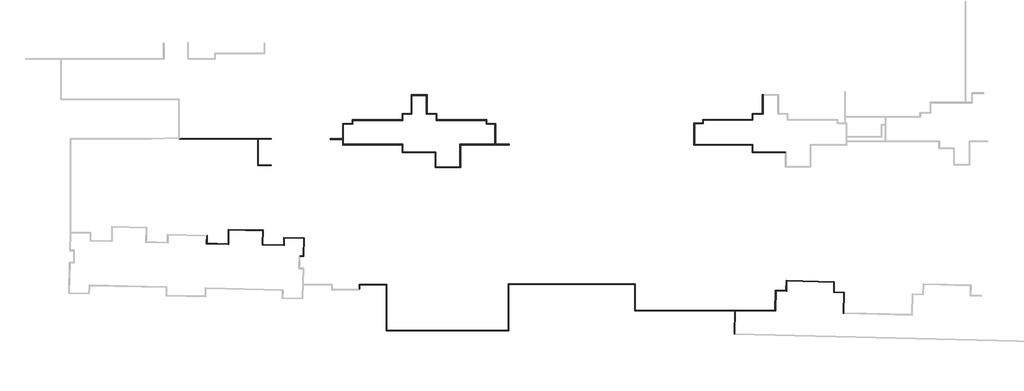
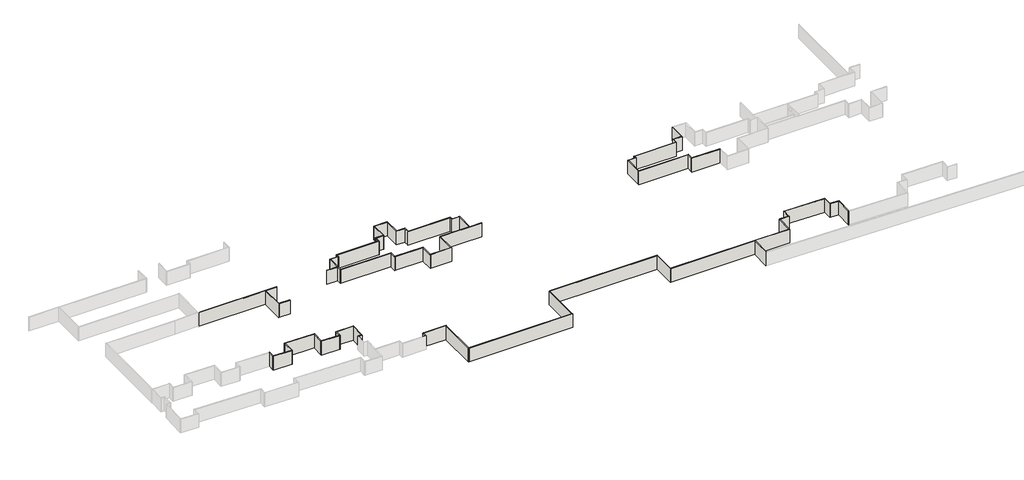
# One storey, part 2 of 8: 62 walls.
"""IFC4 building model written with IfcOpenShell, lengths in millimetres."""

import ifcopenshell
import ifcopenshell.guid

model = None  # the IFC model being written
_history = None  # IfcOwnerHistory: only IFC2X3 demands one
_inside = {}  # id of a spatial element -> (the spatial element, [elements in it])
_under = {}  # id of a project, library or spatial element -> (it, [spatial elements below it])
_declared = {}  # id of a project -> (the project, [libraries it declares])
_typed = {}  # id of a type object -> (the type object, [elements of that type])
_made_of = {}  # id of a material, layer set ... -> (it, [elements and type objects made of it])


def new_model(schema):
    """Start an empty IFC model of exactly this schema.

    Asked for "IFC4X3", IfcOpenShell would pick the latest addendum, in which some entities
    have other attributes; the version numbers below select the first issue.
    IFC2X3 requires an IfcOwnerHistory on every rooted entity: one is made here for all.
    """
    global model, _history
    if schema == "IFC4X3":
        model = ifcopenshell.file(schema_version=(4, 3, 0, 0))
    else:
        model = ifcopenshell.file(schema=schema)
    _inside.clear()
    _under.clear()
    _declared.clear()
    _typed.clear()
    _made_of.clear()
    _history = None
    if model.schema == "IFC2X3":
        org = make("IfcOrganization", Name="unknown")
        user = make(
            "IfcPersonAndOrganization",
            ThePerson=make("IfcPerson", FamilyName="unknown"),
            TheOrganization=org,
        )
        app = make(
            "IfcApplication",
            ApplicationDeveloper=org,
            Version="unknown",
            ApplicationFullName="unknown",
            ApplicationIdentifier="unknown",
        )
        _history = make(
            "IfcOwnerHistory",
            OwningUser=user,
            OwningApplication=app,
            ChangeAction="ADDED",
            CreationDate=0,
        )
    return model


def make(cls, **values):
    """One entity of the class cls with the attributes given. An attribute that is None is left unset."""
    return model.create_entity(
        cls, **{name: value for name, value in values.items() if value is not None}
    )


def rooted(cls, **values):
    """An entity with a GlobalId (a new one), such as an element, a storey or a relation."""
    return make(cls, GlobalId=ifcopenshell.guid.new(), OwnerHistory=_history, **values)


def si_unit(unit_type, name, prefix=None):
    """IfcSIUnit, for example si_unit("LENGTHUNIT", "METRE", prefix="MILLI")."""
    return make("IfcSIUnit", UnitType=unit_type, Prefix=prefix, Name=name)


def assignment(units):
    """IfcUnitAssignment: the units of a project."""
    return None if units is None else make("IfcUnitAssignment", Units=units)


def point(xyz):
    """IfcCartesianPoint."""
    return None if xyz is None else make("IfcCartesianPoint", Coordinates=xyz)


def direction(xyz):
    """IfcDirection."""
    return None if xyz is None else make("IfcDirection", DirectionRatios=xyz)


def frame(location, z_axis=None, x_axis=None):
    """IfcAxis2Placement3D, a coordinate frame: its origin and axes. An axis left out is left unset."""
    return make(
        "IfcAxis2Placement3D",
        Location=point(location),
        Axis=direction(z_axis),
        RefDirection=direction(x_axis),
    )


def origin():
    """The frame at (0, 0, 0) with its axes left unset."""
    return frame((0.0, 0.0, 0.0))


def origin_with_axes():
    """The frame at (0, 0, 0) with the z axis (0, 0, 1) and the x axis (1, 0, 0) written out."""
    return frame((0.0, 0.0, 0.0), z_axis=(0.0, 0.0, 1.0), x_axis=(1.0, 0.0, 0.0))


def place(relative_to, where):
    """IfcLocalPlacement: puts the frame where relative to a parent placement (None: the world)."""
    return make(
        "IfcLocalPlacement", PlacementRelTo=relative_to, RelativePlacement=where
    )


def context(
    kind, dimensions, precision=None, world=None, true_north=None, identifier=None
):
    """IfcGeometricRepresentationContext, for example the 3D "Model" context."""
    return make(
        "IfcGeometricRepresentationContext",
        ContextIdentifier=identifier,
        ContextType=kind,
        CoordinateSpaceDimension=dimensions,
        Precision=precision,
        WorldCoordinateSystem=world,
        TrueNorth=true_north,
    )


def project(units=None, contexts=None):
    """IfcProject with its units and contexts."""
    return rooted(
        "IfcProject",
        Name="project",
        RepresentationContexts=contexts,
        UnitsInContext=assignment(units),
    )


def spatial(cls, under=None, at=None, **own):
    """A site, building, storey or space (cls), placed at a placement, below another one or the project."""
    s = rooted(cls, ObjectPlacement=at, **own)
    if under is not None:
        _under.setdefault(under.id(), (under, []))[1].append(s)
    return s


def polyline(points):
    """IfcPolyline through the points."""
    return make("IfcPolyline", Points=[point(p) for p in points])


def outline(outer, holes=None, kind="AREA"):
    """IfcArbitraryClosedProfileDef: a profile drawn as a closed curve; with holes, ...WithVoids."""
    if holes is None:
        return make("IfcArbitraryClosedProfileDef", ProfileType=kind, OuterCurve=outer)
    return make(
        "IfcArbitraryProfileDefWithVoids",
        ProfileType=kind,
        OuterCurve=outer,
        InnerCurves=holes,
    )


def extrude(swept, where, along, depth):
    """IfcExtrudedAreaSolid: the profile swept, set in the frame where, extruded along a direction by depth."""
    return make(
        "IfcExtrudedAreaSolid",
        SweptArea=swept,
        Position=where,
        ExtrudedDirection=direction(along),
        Depth=depth,
    )


def faces_of(points, faces, orient=None, outer=None):
    """IfcFace entities. A face is a list of loops; a loop is a list of indices into points, from 0.

    orient and outer hold one flag for each loop. By default every Orientation is true, the
    first loop of a face is its IfcFaceOuterBound and the others are IfcFaceBound.
    """
    made = []
    for i, loops in enumerate(faces):
        bounds = []
        for j, loop in enumerate(loops):
            is_outer = j == 0 if outer is None else outer[i][j]
            bounds.append(
                make(
                    "IfcFaceOuterBound" if is_outer else "IfcFaceBound",
                    Bound=make("IfcPolyLoop", Polygon=[points[k] for k in loop]),
                    Orientation=True if orient is None else orient[i][j],
                )
            )
        made.append(make("IfcFace", Bounds=bounds))
    return made


def faceted_brep(points, faces, orient=None, outer=None, voids=None):
    """IfcFacetedBrep: a solid bounded by flat faces; with voids (closed shells), ...WithVoids."""
    shared = [point(p) for p in points]
    hull = make("IfcClosedShell", CfsFaces=faces_of(shared, faces, orient, outer))
    if voids is None:
        return make("IfcFacetedBrep", Outer=hull)
    return make(
        "IfcFacetedBrepWithVoids",
        Outer=hull,
        Voids=[
            make(cls, CfsFaces=faces_of(shared, fs, o, b)) for cls, fs, o, b in voids
        ],
    )


def shape(context_of_items, identifier, shape_type, items):
    """IfcShapeRepresentation: the items that make up one representation, for example the "Body"."""
    return make(
        "IfcShapeRepresentation",
        ContextOfItems=context_of_items,
        RepresentationIdentifier=identifier,
        RepresentationType=shape_type,
        Items=items,
    )


def made_of(thing, what):
    """Note that an element or type object is made of a material, layer set ...; save() writes the relation."""
    if what is not None:
        _made_of.setdefault(what.id(), (what, []))[1].append(thing)
    return thing


def element(
    cls,
    number,
    at=None,
    inside=None,
    cuts=None,
    type_object=None,
    material=None,
    context=None,
    identifier="Body",
    shape_type=None,
    held_by="IfcProductDefinitionShape",
    body=None,
    shapes=None,
    **own,
):
    """One element of the class cls, such as IfcWall. Its Tag is "e" and its number.

    at: its placement. inside: the storey or other place that contains it. cuts: it is an
    opening in that element (IfcRelVoidsElement). A single representation is given by context,
    identifier, shape_type and body (its items); several are given by shapes. held_by: the class
    of the entity that holds the representations. save() writes the other relations.
    """
    e = rooted(cls, Tag="e%d" % number, ObjectPlacement=at, **own)
    if body is not None:
        shapes = [shape(context, identifier, shape_type, body)]
    if shapes is not None:
        e.Representation = make(held_by, Representations=shapes)
    if inside is not None:
        _inside.setdefault(inside.id(), (inside, []))[1].append(e)
    if cuts is not None:
        rooted(
            "IfcRelVoidsElement", RelatingBuildingElement=cuts, RelatedOpeningElement=e
        )
    if type_object is not None:
        _typed.setdefault(type_object.id(), (type_object, []))[1].append(e)
    return made_of(e, material)


def aggregate(whole, parts):
    """IfcRelAggregates: a whole, such as a stair, and the parts it consists of."""
    return rooted("IfcRelAggregates", RelatingObject=whole, RelatedObjects=parts)


def save(model, path):
    """Write the relations noted so far, then the file.

    IfcRelAggregates (storeys below a building ...), IfcRelContainedInSpatialStructure (elements
    in a storey), IfcRelDefinesByType, IfcRelAssociatesMaterial and IfcRelDeclares: one each for
    every whole, place, type object, material and project.
    """
    for whole, parts in _under.values():
        aggregate(whole, parts)
    for where, things in _inside.values():
        rooted(
            "IfcRelContainedInSpatialStructure",
            RelatedElements=things,
            RelatingStructure=where,
        )
    for kind, things in _typed.values():
        rooted("IfcRelDefinesByType", RelatedObjects=things, RelatingType=kind)
    for what, things in _made_of.values():
        rooted("IfcRelAssociatesMaterial", RelatedObjects=things, RelatingMaterial=what)
    for by, libraries in _declared.values():
        rooted("IfcRelDeclares", RelatingContext=by, RelatedDefinitions=libraries)
    model.write(path)


model = new_model("IFC4")

# Units and contexts
model_context = context("Model", 3, world=origin())
ifc_project = project(units=[si_unit("LENGTHUNIT", "METRE", prefix="MILLI")], contexts=[model_context])

# Site, building, storey
site = spatial("IfcSite", under=ifc_project)
building = spatial("IfcBuilding", under=site)
storey = spatial("IfcBuildingStorey", under=building, Name="户型图", Elevation=0.0)

# Walls
placement = place(None, origin())
element("IfcWall", 1, ObjectType="所有墙体", at=placement, inside=storey, context=model_context, shape_type="Brep", body=[
    faceted_brep([(147810.3217494, 32480.6370168, 0.0), (148610.1884761, 32461.0693182, 0.0), (148610.1884761, 32461.0693182, 3300.0), (147810.3217494, 32480.6370168, 3300.0), (147813.2565152, 32600.6011245, 0.0), (147813.2565152, 32600.6011245, 3300.0), (148493.1591342, 32583.9681917, 3300.0), (148613.1232419, 32581.0334259, 3300.0), (148613.1232419, 32581.0334259, 0.0), (148493.1591342, 32583.9681917, 0.0)], [[[0, 1, 2, 3]], [[4, 5, 6, 7, 8, 9]], [[1, 0, 4, 9, 8]], [[3, 2, 7, 6, 5]], [[0, 3, 5, 4]], [[2, 1, 8, 7]]]),
])
element("IfcWall", 2, ObjectType="所有墙体", at=placement, inside=storey, context=model_context, shape_type="Brep", body=[
    faceted_brep([(148613.1232419, 32581.0334259, 0.0), (148698.7197127, 36079.9512285, 0.0), (148698.7197127, 36079.9512285, 3300.0), (148613.1232419, 32581.0334259, 3300.0), (148493.1591342, 32583.9681917, 0.0), (148493.1591342, 32583.9681917, 3300.0), (148575.8208392, 35962.9218865, 3300.0), (148578.755605, 36082.8859942, 3300.0), (148578.755605, 36082.8859942, 0.0), (148575.8208392, 35962.9218865, 0.0)], [[[0, 1, 2, 3]], [[4, 5, 6, 7, 8, 9]], [[1, 0, 4, 9, 8]], [[3, 2, 7, 6, 5]], [[0, 3, 5, 4]], [[2, 1, 8, 7]]]),
])
element("IfcWall", 3, ObjectType="所有墙体", at=placement, inside=storey, context=model_context, shape_type="Brep", body=[
    faceted_brep([(148578.755605, 36082.8859942, 0.0), (144680.0766894, 36178.2621005, 0.0), (144680.0766894, 36178.2621005, 3300.0), (148578.755605, 36082.8859942, 3300.0), (148575.8208392, 35962.9218865, 0.0), (148575.8208392, 35962.9218865, 3300.0), (144797.1060314, 36055.3632269, 3300.0), (144677.1419237, 36058.2979927, 3300.0), (144677.1419237, 36058.2979927, 0.0), (144797.1060314, 36055.3632269, 0.0)], [[[0, 1, 2, 3]], [[4, 5, 6, 7, 8, 9]], [[1, 0, 4, 9, 8]], [[3, 2, 7, 6, 5]], [[0, 3, 5, 4]], [[2, 1, 8, 7]]]),
])
element("IfcWall", 4, ObjectType="所有墙体", at=placement, inside=storey, context=model_context, shape_type="Brep", body=[
    faceted_brep([(144677.1419237, 36058.2979927, 0.0), (144643.3963311, 34678.8830052, 0.0), (144640.4615653, 34558.9188975, 0.0), (144640.4615653, 34558.9188975, 3300.0), (144643.3963311, 34678.8830052, 3300.0), (144677.1419237, 36058.2979927, 3300.0), (144797.1060314, 36055.3632269, 0.0), (144797.1060314, 36055.3632269, 3300.0), (144760.425673, 34555.9841317, 3300.0), (144760.425673, 34555.9841317, 0.0)], [[[0, 1, 2, 3, 4, 5]], [[6, 7, 8, 9]], [[2, 1, 0, 6, 9]], [[5, 4, 3, 8, 7]], [[0, 5, 7, 6]], [[3, 2, 9, 8]]]),
])
element("IfcWall", 5, ObjectType="所有墙体", at=placement, inside=storey, context=model_context, shape_type="Brep", body=[
    faceted_brep([(144643.3963311, 34678.8830052, 0.0), (140614.5354623, 34777.4438435, 0.0), (140494.5713546, 34780.3786093, 0.0), (140494.5713546, 34780.3786093, 3300.0), (140614.5354623, 34777.4438435, 3300.0), (144643.3963311, 34678.8830052, 3300.0), (144640.4615653, 34558.9188975, 0.0), (144640.4615653, 34558.9188975, 3300.0), (140491.6365888, 34660.4145015, 3300.0), (140491.6365888, 34660.4145015, 0.0)], [[[0, 1, 2, 3, 4, 5]], [[6, 7, 8, 9]], [[2, 1, 0, 6, 9]], [[5, 4, 3, 8, 7]], [[0, 5, 7, 6]], [[3, 2, 9, 8]]]),
])
element("IfcWall", 6, ObjectType="所有墙体", at=placement, inside=storey, context=model_context, shape_type="Brep", body=[
    faceted_brep([(140614.5354623, 34777.4438435, 0.0), (140683.0178151, 37576.7896669, 0.0), (140683.0178151, 37576.7896669, 3300.0), (140614.5354623, 34777.4438435, 3300.0), (140494.5713546, 34780.3786093, 0.0), (140494.5713546, 34780.3786093, 3300.0), (140560.1189415, 37459.760325, 3300.0), (140563.0537073, 37579.7244327, 3300.0), (140563.0537073, 37579.7244327, 0.0), (140560.1189415, 37459.760325, 0.0)], [[[0, 1, 2, 3]], [[4, 5, 6, 7, 8, 9]], [[1, 0, 4, 9, 8]], [[3, 2, 7, 6, 5]], [[0, 3, 5, 4]], [[2, 1, 8, 7]]]),
])
element("IfcWall", 7, ObjectType="所有墙体", at=placement, inside=storey, context=model_context, shape_type="Brep", body=[
    faceted_brep([(140563.0537073, 37579.7244327, 0.0), (133863.6960372, 37743.6155001, 0.0), (133863.6960372, 37743.6155001, 3300.0), (140563.0537073, 37579.7244327, 3300.0), (140560.1189415, 37459.760325, 0.0), (140560.1189415, 37459.760325, 3300.0), (133983.6960372, 37620.6439532, 3300.0), (133863.6960372, 37623.5795971, 3300.0), (133863.6960372, 37623.5795971, 0.0), (133983.6960372, 37620.6439532, 0.0)], [[[0, 1, 2, 3]], [[4, 5, 6, 7, 8, 9]], [[1, 0, 4, 9, 8]], [[3, 2, 7, 6, 5]], [[0, 3, 5, 4]], [[2, 1, 8, 7]]]),
])
element("IfcWall", 8, ObjectType="所有墙体", at=placement, inside=storey, context=model_context, shape_type="Brep", body=[
    faceted_brep([(133863.6960372, 37623.5795971, 0.0), (133863.6960372, 34942.594345, 0.0), (133863.6960372, 34822.558442, 0.0), (133863.6960372, 34822.558442, 3300.0), (133863.6960372, 34942.594345, 3300.0), (133863.6960372, 37623.5795971, 3300.0), (133983.6960372, 37620.6439532, 0.0), (133983.6960372, 37620.6439532, 3300.0), (133983.6960372, 34819.6227982, 3300.0), (133983.6960372, 34819.6227982, 0.0)], [[[0, 1, 2, 3, 4, 5]], [[6, 7, 8, 9]], [[2, 1, 0, 6, 9]], [[5, 4, 3, 8, 7]], [[0, 5, 7, 6]], [[3, 2, 9, 8]]]),
])
element("IfcWall", 9, ObjectType="所有墙体", at=placement, inside=storey, context=model_context, shape_type="Brep", body=[
    faceted_brep([(133863.6960372, 34942.594345, 0.0), (129767.3964735, 35042.8049832, 0.0), (129647.4323657, 35045.739749, 0.0), (129647.4323657, 35045.739749, 3300.0), (129767.3964735, 35042.8049832, 3300.0), (133863.6960372, 34942.594345, 3300.0), (133863.6960372, 34822.558442, 0.0), (133863.6960372, 34822.558442, 3300.0), (129644.4975999, 34925.7756412, 3300.0), (129644.4975999, 34925.7756412, 0.0)], [[[0, 1, 2, 3, 4, 5]], [[6, 7, 8, 9]], [[2, 1, 0, 6, 9]], [[5, 4, 3, 8, 7]], [[0, 5, 7, 6]], [[3, 2, 9, 8]]]),
])
element("IfcWall", 10, ObjectType="所有墙体", at=placement, inside=storey, context=model_context, shape_type="Brep", body=[
    faceted_brep([(129767.3964735, 35042.8049832, 0.0), (129804.0972544, 36543.0188892, 0.0), (129804.0972544, 36543.0188892, 3300.0), (129767.3964735, 35042.8049832, 3300.0), (129647.4323657, 35045.739749, 0.0), (129647.4323657, 35045.739749, 3300.0), (129681.1983809, 36425.9895472, 3300.0), (129684.1331467, 36545.953655, 3300.0), (129684.1331467, 36545.953655, 0.0), (129681.1983809, 36425.9895472, 0.0)], [[[0, 1, 2, 3]], [[4, 5, 6, 7, 8, 9]], [[1, 0, 4, 9, 8]], [[3, 2, 7, 6, 5]], [[0, 3, 5, 4]], [[2, 1, 8, 7]]]),
])
element("IfcWall", 11, ObjectType="所有墙体", at=placement, inside=storey, context=model_context, shape_type="Brep", body=[
    faceted_brep([(139640.2139729, 55332.5925367, 0.0), (139640.2139729, 50107.6336553, 0.0), (139640.2139729, 50107.6336553, 3300.0), (139640.2139729, 55332.5925367, 3300.0), (139760.2139729, 55332.5925367, 0.0), (139760.2139729, 55332.5925367, 3300.0), (139760.2139729, 50227.6336553, 3300.0), (139760.2139729, 50107.6336553, 3300.0), (139760.2139729, 50107.6336553, 0.0), (139760.2139729, 50227.6336553, 0.0)], [[[0, 1, 2, 3]], [[4, 5, 6, 7, 8, 9]], [[1, 0, 4, 9, 8]], [[3, 2, 7, 6, 5]], [[2, 1, 8, 7]], [[0, 3, 5, 4]]]),
])
element("IfcWall", 12, ObjectType="所有墙体", at=placement, inside=storey, context=model_context, shape_type="SweptSolid", body=[
    extrude(outline(polyline([(142300.2032763, 50107.6336553), (139760.2139729, 50107.6336553), (139760.2139729, 50227.6336553), (142300.2032763, 50227.6336553), (142300.2032763, 50107.6336553)])), origin_with_axes(), (0.0, 0.0, 1.0), 3300.0),
])
element("IfcWall", 13, ObjectType="所有墙体", at=placement, inside=storey, context=model_context, shape_type="Brep", body=[
    faceted_brep([(142300.2032763, 55452.5925367, 0.0), (124545.05609, 55452.5925367, 0.0), (124545.05609, 55452.5925367, 3300.0), (142150.2032763, 55452.5925367, 3300.0), (142300.2032763, 55452.5925367, 3300.0), (142300.2032763, 55452.5925367, 2700.0), (142300.2032763, 55332.5925367, 0.0), (142300.2032763, 55332.5925367, 2700.0), (142300.2032763, 55332.5925367, 3300.0), (142150.2032763, 55332.5925367, 3300.0), (139760.2139729, 55332.5925367, 3300.0), (139640.2139729, 55332.5925367, 3300.0), (134650.2032763, 55332.5925367, 3300.0), (134350.2032763, 55332.5925367, 3300.0), (124425.05609, 55332.5925367, 3300.0), (124425.05609, 55332.5925367, 0.0), (139640.2139729, 55332.5925367, 0.0), (139760.2139729, 55332.5925367, 0.0)], [[[0, 1, 2, 3, 4, 5]], [[6, 7, 8, 9, 10, 11, 12, 13, 14, 15, 16, 17]], [[1, 0, 6, 17, 16, 15]], [[4, 3, 2, 14, 13, 12, 11, 10, 9, 8]], [[0, 5, 4, 8, 7, 6]], [[2, 1, 15, 14]]]),
])
element("IfcWall", 14, ObjectType="所有墙体", at=placement, inside=storey, context=model_context, shape_type="Brep", body=[
    faceted_brep([(159492.7804968, 26052.2214543, 0.0), (159492.7804968, 26924.9842098, 0.0), (159492.7804968, 27044.9842098, 0.0), (159492.7804968, 27044.9842098, 3300.0), (159492.7804968, 26924.9842098, 3300.0), (159492.7804968, 26052.2214543, 3300.0), (159372.7804968, 26052.2214543, 0.0), (159372.7804968, 26052.2214543, 3300.0), (159372.7804968, 27016.5295438, 3300.0), (159372.7804968, 27044.9842098, 3300.0), (159372.7804968, 27044.9842098, 2700.0), (159372.7804968, 27044.9842098, 0.0)], [[[0, 1, 2, 3, 4, 5]], [[6, 7, 8, 9, 10, 11]], [[2, 1, 0, 6, 11]], [[5, 4, 3, 9, 8, 7]], [[0, 5, 7, 6]], [[3, 2, 11, 10, 9]]]),
])
element("IfcWall", 15, ObjectType="所有墙体", at=placement, inside=storey, context=model_context, shape_type="Brep", body=[
    faceted_brep([(159492.7804968, 26924.9842098, 0.0), (164572.7804968, 26924.9842098, 0.0), (164692.7804968, 26924.9842098, 0.0), (164692.7804968, 26924.9842098, 3300.0), (164572.7804968, 26924.9842098, 3300.0), (159492.7804968, 26924.9842098, 3300.0), (159492.7804968, 27044.9842098, 0.0), (159492.7804968, 27044.9842098, 3300.0), (159549.7804968, 27044.9842098, 3300.0), (164692.7804968, 27044.9842098, 3300.0), (164692.7804968, 27044.9842098, 0.0)], [[[0, 1, 2, 3, 4, 5]], [[6, 7, 8, 9, 10]], [[2, 1, 0, 6, 10]], [[5, 4, 3, 9, 8, 7]], [[0, 5, 7, 6]], [[3, 2, 10, 9]]]),
])
element("IfcWall", 16, ObjectType="所有墙体", at=placement, inside=storey, context=model_context, shape_type="Brep", body=[
    faceted_brep([(164572.7804968, 26924.9842098, 0.0), (164572.7804968, 17982.1039685, 0.0), (164572.7804968, 17982.1039685, 3300.0), (164572.7804968, 26924.9842098, 3300.0), (164692.7804968, 26924.9842098, 0.0), (164692.7804968, 26924.9842098, 3300.0), (164692.7804968, 18102.1039685, 3300.0), (164692.7804968, 17982.1039685, 3300.0), (164692.7804968, 17982.1039685, 0.0), (164692.7804968, 18102.1039685, 0.0)], [[[0, 1, 2, 3]], [[4, 5, 6, 7, 8, 9]], [[1, 0, 4, 9, 8]], [[3, 2, 7, 6, 5]], [[0, 3, 5, 4]], [[2, 1, 8, 7]]]),
])
element("IfcWall", 17, ObjectType="所有墙体", at=placement, inside=storey, context=model_context, shape_type="Brep", body=[
    faceted_brep([(164692.7804968, 17982.1039685, 0.0), (188424.7804971, 17982.1039685, 0.0), (188424.7804971, 17982.1039685, 3300.0), (164692.7804968, 17982.1039685, 3300.0), (164692.7804968, 18102.1039685, 0.0), (164692.7804968, 18102.1039685, 3300.0), (188304.7804971, 18102.1039685, 3300.0), (188424.7804971, 18102.1039685, 3300.0), (188424.7804971, 18102.1039685, 0.0), (188304.7804971, 18102.1039685, 0.0)], [[[0, 1, 2, 3]], [[4, 5, 6, 7, 8, 9]], [[1, 0, 4, 9, 8]], [[3, 2, 7, 6, 5]], [[0, 3, 5, 4]], [[2, 1, 8, 7]]]),
])
element("IfcWall", 18, ObjectType="所有墙体", at=placement, inside=storey, context=model_context, shape_type="Brep", body=[
    faceted_brep([(188424.7804971, 18102.1039685, 0.0), (188424.7804971, 26982.1039685, 0.0), (188424.7804971, 27102.1039685, 0.0), (188424.7804971, 27102.1039685, 3300.0), (188424.7804971, 26982.1039685, 3300.0), (188424.7804971, 18102.1039685, 3300.0), (188304.7804971, 18102.1039685, 0.0), (188304.7804971, 18102.1039685, 3300.0), (188304.7804971, 26942.26105, 3300.0), (188304.7804971, 27102.1039685, 3300.0), (188304.7804971, 27102.1039685, 2700.0), (188304.7804971, 27102.1039685, 0.0), (188349.7804968, 27102.1039685, 3300.0)], [[[0, 1, 2, 3, 4, 5]], [[6, 7, 8, 9, 10, 11]], [[2, 1, 0, 6, 11]], [[5, 4, 3, 12, 9, 8, 7]], [[0, 5, 7, 6]], [[3, 2, 11, 10, 9, 12]]]),
])
element("IfcWall", 19, ObjectType="所有墙体", at=placement, inside=storey, context=model_context, shape_type="Brep", body=[
    faceted_brep([(188424.7804971, 26982.1039685, 0.0), (212939.7704217, 26982.1039685, 0.0), (213059.7704217, 26982.1039685, 0.0), (213059.7704217, 26982.1039685, 3300.0), (212939.7704217, 26982.1039685, 3300.0), (188424.7804971, 26982.1039685, 3300.0), (188424.7804971, 27102.1039685, 0.0), (188424.7804971, 27102.1039685, 3300.0), (212939.7704217, 27102.1039685, 3300.0), (213059.7704217, 27102.1039685, 3300.0), (213059.7704217, 27102.1039685, 2700.0), (213059.7704217, 27102.1039685, 0.0)], [[[0, 1, 2, 3, 4, 5]], [[6, 7, 8, 9, 10, 11]], [[2, 1, 0, 6, 11]], [[5, 4, 3, 9, 8, 7]], [[0, 5, 7, 6]], [[3, 2, 11, 10, 9]]]),
])
element("IfcWall", 20, ObjectType="所有墙体", at=placement, inside=storey, context=model_context, shape_type="Brep", body=[
    faceted_brep([(212939.7704217, 26982.1039685, 0.0), (212939.7704217, 21832.0972046, 0.0), (212939.7704217, 21832.0972046, 3300.0), (212939.7704217, 26982.1039685, 3300.0), (213059.7704217, 26982.1039685, 0.0), (213059.7704217, 26982.1039685, 3300.0), (213059.7704217, 21952.0972046, 3300.0), (213059.7704217, 21832.0972046, 3300.0), (213059.7704217, 21832.0972046, 0.0), (213059.7704217, 21952.0972046, 0.0)], [[[0, 1, 2, 3]], [[4, 5, 6, 7, 8, 9]], [[1, 0, 4, 9, 8]], [[3, 2, 7, 6, 5]], [[0, 3, 5, 4]], [[2, 1, 8, 7]]]),
])
element("IfcWall", 21, ObjectType="所有墙体", at=placement, inside=storey, context=model_context, shape_type="Brep", body=[
    faceted_brep([(213059.7704217, 21832.0972046, 0.0), (232368.9498192, 21832.0972046, 0.0), (232488.9860236, 21832.0972046, 0.0), (240288.4203946, 21832.0972046, 0.0), (240288.4203946, 21832.0972046, 3300.0), (232488.9860236, 21832.0972046, 3300.0), (232368.9498192, 21832.0972046, 3300.0), (213059.7704217, 21832.0972046, 3300.0), (213059.7704217, 21952.0972046, 0.0), (213059.7704217, 21952.0972046, 3300.0), (240171.3321364, 21952.0972046, 3300.0), (240291.3683409, 21952.0972046, 3300.0), (240291.3683409, 21952.0972046, 0.0), (240171.3321364, 21952.0972046, 0.0)], [[[0, 1, 2, 3, 4, 5, 6, 7]], [[8, 9, 10, 11, 12, 13]], [[3, 2, 1, 0, 8, 13, 12]], [[7, 6, 5, 4, 11, 10, 9]], [[0, 7, 9, 8]], [[4, 3, 12, 11]]]),
])
element("IfcWall", 22, ObjectType="所有墙体", at=placement, inside=storey, context=model_context, shape_type="Brep", body=[
    faceted_brep([(240291.3683409, 21952.0972046, 0.0), (240384.6551744, 25749.4594497, 0.0), (240387.6022316, 25869.4232561, 0.0), (240387.6022316, 25869.4232561, 3300.0), (240384.6551744, 25749.4594497, 3300.0), (240291.3683409, 21952.0972046, 3300.0), (240171.3321364, 21952.0972046, 0.0), (240171.3321364, 21952.0972046, 3300.0), (240267.6384252, 25872.3703133, 3300.0), (240267.6384252, 25872.3703133, 0.0)], [[[0, 1, 2, 3, 4, 5]], [[6, 7, 8, 9]], [[2, 1, 0, 6, 9]], [[5, 4, 3, 8, 7]], [[3, 2, 9, 8]], [[0, 5, 7, 6]]]),
])
element("IfcWall", 23, ObjectType="所有墙体", at=placement, inside=storey, context=model_context, shape_type="Brep", body=[
    faceted_brep([(240384.6551744, 25749.4594497, 0.0), (242434.0834863, 25699.1127444, 0.0), (242434.0834863, 25699.1127444, 3300.0), (240384.6551744, 25749.4594497, 3300.0), (240387.6022316, 25869.4232561, 0.0), (240387.6022316, 25869.4232561, 3300.0), (242317.0667371, 25822.023608, 3300.0), (242437.0305435, 25819.0765508, 3300.0), (242437.0305435, 25819.0765508, 0.0), (242317.0667371, 25822.023608, 0.0)], [[[0, 1, 2, 3]], [[4, 5, 6, 7, 8, 9]], [[1, 0, 4, 9, 8]], [[3, 2, 7, 6, 5]], [[0, 3, 5, 4]], [[2, 1, 8, 7]]]),
])
element("IfcWall", 24, ObjectType="所有墙体", at=placement, inside=storey, context=model_context, shape_type="Brep", body=[
    faceted_brep([(242437.0305435, 25819.0765508, 0.0), (242482.197099, 27657.640106, 0.0), (242485.1441561, 27777.6039124, 0.0), (242485.1441561, 27777.6039124, 3300.0), (242482.197099, 27657.640106, 3300.0), (242437.0305435, 25819.0765508, 3300.0), (242317.0667371, 25822.023608, 0.0), (242317.0667371, 25822.023608, 3300.0), (242365.1803497, 27780.5509696, 3300.0), (242365.1803497, 27780.5509696, 0.0)], [[[0, 1, 2, 3, 4, 5]], [[6, 7, 8, 9]], [[2, 1, 0, 6, 9]], [[5, 4, 3, 8, 7]], [[0, 5, 7, 6]], [[3, 2, 9, 8]]]),
])
element("IfcWall", 25, ObjectType="所有墙体", at=placement, inside=storey, context=model_context, shape_type="Brep", body=[
    faceted_brep([(242482.197099, 27657.640106, 0.0), (251561.2137426, 27434.6029923, 0.0), (251681.2137426, 27431.655046, 0.0), (251681.2137426, 27431.655046, 3300.0), (251561.2137426, 27434.6029923, 3300.0), (242482.197099, 27657.640106, 3300.0), (242485.1441561, 27777.6039124, 0.0), (242485.1441561, 27777.6039124, 3300.0), (251681.2137426, 27551.6912505, 3300.0), (251681.2137426, 27551.6912505, 0.0)], [[[0, 1, 2, 3, 4, 5]], [[6, 7, 8, 9]], [[2, 1, 0, 6, 9]], [[5, 4, 3, 8, 7]], [[0, 5, 7, 6]], [[3, 2, 9, 8]]]),
])
element("IfcWall", 26, ObjectType="所有墙体", at=placement, inside=storey, context=model_context, shape_type="Brep", body=[
    faceted_brep([(251561.2137426, 27434.6029923, 0.0), (251561.2137426, 25434.6029923, 0.0), (251561.2137426, 25434.6029923, 3300.0), (251561.2137426, 27434.6029923, 3300.0), (251681.2137426, 27431.655046, 0.0), (251681.2137426, 27431.655046, 3300.0), (251681.2137426, 25551.6912505, 3300.0), (251681.2137426, 25431.655046, 3300.0), (251681.2137426, 25431.655046, 0.0), (251681.2137426, 25551.6912505, 0.0)], [[[0, 1, 2, 3]], [[4, 5, 6, 7, 8, 9]], [[1, 0, 4, 9, 8]], [[3, 2, 7, 6, 5]], [[0, 3, 5, 4]], [[2, 1, 8, 7]]]),
])
element("IfcWall", 27, ObjectType="所有墙体", at=placement, inside=storey, context=model_context, shape_type="Brep", body=[
    faceted_brep([(251681.2137426, 25431.655046, 0.0), (253560.0154882, 25385.4999904, 0.0), (253679.9792946, 25382.5529332, 0.0), (253679.9792946, 25382.5529332, 3300.0), (253560.0154882, 25385.4999904, 3300.0), (251681.2137426, 25431.655046, 3300.0), (251681.2137426, 25551.6912505, 0.0), (251681.2137426, 25551.6912505, 3300.0), (253682.9263518, 25502.5167396, 3300.0), (253682.9263518, 25502.5167396, 0.0)], [[[0, 1, 2, 3, 4, 5]], [[6, 7, 8, 9]], [[2, 1, 0, 6, 9]], [[5, 4, 3, 8, 7]], [[0, 5, 7, 6]], [[3, 2, 9, 8]]]),
])
element("IfcWall", 28, ObjectType="所有墙体", at=placement, inside=storey, context=model_context, shape_type="Brep", body=[
    faceted_brep([(253560.0154882, 25385.4999904, 0.0), (253461.2890729, 21366.7124748, 0.0), (253461.2890729, 21366.7124748, 3300.0), (253560.0154882, 25385.4999904, 3300.0), (253679.9792946, 25382.5529332, 0.0), (253679.9792946, 25382.5529332, 3300.0), (253584.1999365, 21483.7292241, 3300.0), (253581.2528793, 21363.7654177, 3300.0), (253581.2528793, 21363.7654177, 0.0), (253584.1999365, 21483.7292241, 0.0)], [[[0, 1, 2, 3]], [[4, 5, 6, 7, 8, 9]], [[1, 0, 4, 9, 8]], [[3, 2, 7, 6, 5]], [[0, 3, 5, 4]], [[2, 1, 8, 7]]]),
])
element("IfcWall", 29, ObjectType="所有墙体", at=placement, inside=storey, context=model_context, shape_type="SweptSolid", body=[
    extrude(outline(polyline([(232488.9860236, 21832.0972046), (232379.4299892, 17372.4759146), (232259.4661827, 17375.4229718), (232368.9498192, 21832.0972046), (232488.9860236, 21832.0972046)])), origin_with_axes(), (0.0, 0.0, 1.0), 3300.0),
])
element("IfcWall", 30, ObjectType="所有墙体", at=placement, inside=storey, context=model_context, shape_type="Brep", body=[
    faceted_brep([(242218.4382799, 52813.0860808, 0.0), (235838.4382799, 52813.0860808, 0.0), (235718.4382799, 52813.0860808, 0.0), (235718.4382799, 52813.0860808, 3300.0), (235838.4382799, 52813.0860808, 3300.0), (242218.4382799, 52813.0860808, 3300.0), (242218.4382799, 52693.0860808, 0.0), (242218.4382799, 52693.0860808, 3300.0), (235718.4382799, 52693.0860808, 3300.0), (235718.4382799, 52693.0860808, 0.0)], [[[0, 1, 2, 3, 4, 5]], [[6, 7, 8, 9]], [[2, 1, 0, 6, 9]], [[5, 4, 3, 8, 7]], [[0, 5, 7, 6]], [[3, 2, 9, 8]]]),
])
element("IfcWall", 31, ObjectType="所有墙体", at=placement, inside=storey, context=model_context, shape_type="Brep", body=[
    faceted_brep([(235838.4382799, 52813.0860808, 0.0), (235838.4382799, 54252.3246977, 0.0), (235838.4382799, 54252.3246977, 3300.0), (235838.4382799, 52813.0860808, 3300.0), (235718.4382799, 52813.0860808, 0.0), (235718.4382799, 52813.0860808, 3300.0), (235718.4382799, 54132.3246977, 3300.0), (235718.4382799, 54252.3246977, 3300.0), (235718.4382799, 54252.3246977, 0.0), (235718.4382799, 54132.3246977, 0.0)], [[[0, 1, 2, 3]], [[4, 5, 6, 7, 8, 9]], [[1, 0, 4, 9, 8]], [[3, 2, 7, 6, 5]], [[0, 3, 5, 4]], [[2, 1, 8, 7]]]),
])
element("IfcWall", 32, ObjectType="所有墙体", at=placement, inside=storey, context=model_context, shape_type="Brep", body=[
    faceted_brep([(235718.4382799, 54252.3246977, 0.0), (224538.4382799, 54252.3246977, 0.0), (224418.4382799, 54252.3246977, 0.0), (224418.4382799, 54252.3246977, 3300.0), (224538.4382799, 54252.3246977, 3300.0), (235718.4382799, 54252.3246977, 3300.0), (235718.4382799, 54132.3246977, 0.0), (235718.4382799, 54132.3246977, 3300.0), (224418.4382799, 54132.3246977, 3300.0), (224418.4382799, 54132.3246977, 0.0)], [[[0, 1, 2, 3, 4, 5]], [[6, 7, 8, 9]], [[2, 1, 0, 6, 9]], [[5, 4, 3, 8, 7]], [[0, 5, 7, 6]], [[3, 2, 9, 8]]]),
])
element("IfcWall", 33, ObjectType="所有墙体", at=placement, inside=storey, context=model_context, shape_type="Brep", body=[
    faceted_brep([(224538.4382799, 54252.3246977, 0.0), (224538.4382799, 58332.3246977, 0.0), (224538.4382799, 58452.3246977, 0.0), (224538.4382799, 58452.3246977, 3300.0), (224538.4382799, 58332.3246977, 3300.0), (224538.4382799, 54252.3246977, 3300.0), (224418.4382799, 54252.3246977, 0.0), (224418.4382799, 54252.3246977, 3300.0), (224418.4382799, 58452.3246977, 3300.0), (224418.4382799, 58452.3246977, 0.0)], [[[0, 1, 2, 3, 4, 5]], [[6, 7, 8, 9]], [[2, 1, 0, 6, 9]], [[5, 4, 3, 8, 7]], [[0, 5, 7, 6]], [[3, 2, 9, 8]]]),
])
element("IfcWall", 34, ObjectType="所有墙体", at=placement, inside=storey, context=model_context, shape_type="Brep", body=[
    faceted_brep([(224538.4382799, 58332.3246977, 0.0), (226259.8021768, 58332.3246977, 0.0), (226259.8021768, 58332.3246977, 3300.0), (224538.4382799, 58332.3246977, 3300.0), (224538.4382799, 58452.3246977, 0.0), (224538.4382799, 58452.3246977, 3300.0), (226139.8021768, 58452.3246977, 3300.0), (226259.8021768, 58452.3246977, 3300.0), (226259.8021768, 58452.3246977, 0.0), (226139.8021768, 58452.3246977, 0.0)], [[[0, 1, 2, 3]], [[4, 5, 6, 7, 8, 9]], [[1, 0, 4, 9, 8]], [[3, 2, 7, 6, 5]], [[0, 3, 5, 4]], [[2, 1, 8, 7]]]),
])
element("IfcWall", 35, ObjectType="所有墙体", at=placement, inside=storey, context=model_context, shape_type="Brep", body=[
    faceted_brep([(226259.8021768, 58452.3246977, 0.0), (226259.8021768, 58982.2610502, 0.0), (226259.8021768, 59102.2610502, 0.0), (226259.8021768, 59102.2610502, 3300.0), (226259.8021768, 58982.2610502, 3300.0), (226259.8021768, 58452.3246977, 3300.0), (226139.8021768, 58452.3246977, 0.0), (226139.8021768, 58452.3246977, 3300.0), (226139.8021768, 59102.2610502, 3300.0), (226139.8021768, 59102.2610502, 0.0)], [[[0, 1, 2, 3, 4, 5]], [[6, 7, 8, 9]], [[2, 1, 0, 6, 9]], [[5, 4, 3, 8, 7]], [[0, 5, 7, 6]], [[3, 2, 9, 8]]]),
])
element("IfcWall", 36, ObjectType="所有墙体", at=placement, inside=storey, context=model_context, shape_type="Brep", body=[
    faceted_brep([(226259.8021768, 58982.2610502, 0.0), (235838.4382799, 58982.2610502, 0.0), (235838.4382799, 58982.2610502, 3300.0), (226259.8021768, 58982.2610502, 3300.0), (226259.8021768, 59102.2610502, 0.0), (226259.8021768, 59102.2610502, 3300.0), (235718.4382799, 59102.2610502, 3300.0), (235838.4382799, 59102.2610502, 3300.0), (235838.4382799, 59102.2610502, 0.0), (235718.4382799, 59102.2610502, 0.0)], [[[0, 1, 2, 3]], [[4, 5, 6, 7, 8, 9]], [[1, 0, 4, 9, 8]], [[3, 2, 7, 6, 5]], [[0, 3, 5, 4]], [[2, 1, 8, 7]]]),
])
element("IfcWall", 37, ObjectType="所有墙体", at=placement, inside=storey, context=model_context, shape_type="Brep", body=[
    faceted_brep([(235838.4382799, 59102.2610502, 0.0), (235838.4382799, 60182.2610504, 0.0), (235838.4382799, 60302.2610504, 0.0), (235838.4382799, 60302.2610504, 3300.0), (235838.4382799, 60182.2610504, 3300.0), (235838.4382799, 59102.2610502, 3300.0), (235718.4382799, 59102.2610502, 0.0), (235718.4382799, 59102.2610502, 3300.0), (235718.4382799, 60302.2610504, 3300.0), (235718.4382799, 60302.2610504, 0.0)], [[[0, 1, 2, 3, 4, 5]], [[6, 7, 8, 9]], [[2, 1, 0, 6, 9]], [[5, 4, 3, 8, 7]], [[0, 5, 7, 6]], [[3, 2, 9, 8]]]),
])
element("IfcWall", 38, ObjectType="所有墙体", at=placement, inside=storey, context=model_context, shape_type="Brep", body=[
    faceted_brep([(235838.4382799, 60182.2610504, 0.0), (237859.8021767, 60182.2610504, 0.0), (237859.8021767, 60182.2610504, 3300.0), (235838.4382799, 60182.2610504, 3300.0), (235838.4382799, 60302.2610504, 0.0), (235838.4382799, 60302.2610504, 3300.0), (237739.8021767, 60302.2610504, 3300.0), (237859.8021767, 60302.2610504, 3300.0), (237859.8021767, 60302.2610504, 0.0), (237739.8021767, 60302.2610504, 0.0)], [[[0, 1, 2, 3]], [[4, 5, 6, 7, 8, 9]], [[1, 0, 4, 9, 8]], [[3, 2, 7, 6, 5]], [[0, 3, 5, 4]], [[2, 1, 8, 7]]]),
])
element("IfcWall", 39, ObjectType="所有墙体", at=placement, inside=storey, context=model_context, shape_type="Brep", body=[
    faceted_brep([(237859.8021767, 60302.2610504, 0.0), (237859.8021767, 63882.26105, 0.0), (237859.8021767, 64002.26105, 0.0), (237859.8021767, 64002.26105, 3300.0), (237859.8021767, 63882.26105, 3300.0), (237859.8021767, 60302.2610504, 3300.0), (237739.8021767, 60302.2610504, 0.0), (237739.8021767, 60302.2610504, 3300.0), (237739.8021767, 64002.26105, 3300.0), (237739.8021767, 64002.26105, 0.0)], [[[0, 1, 2, 3, 4, 5]], [[6, 7, 8, 9]], [[2, 1, 0, 6, 9]], [[5, 4, 3, 8, 7]], [[0, 5, 7, 6]], [[3, 2, 9, 8]]]),
])
element("IfcWall", 40, ObjectType="所有墙体", at=placement, inside=storey, context=model_context, shape_type="Brep", body=[
    faceted_brep([(156260.298991, 54181.7848082, 0.0), (167685.197808, 54181.7848082, 0.0), (167805.197808, 54181.7848082, 0.0), (167805.197808, 54181.7848082, 3300.0), (167685.197808, 54181.7848082, 3300.0), (156260.298991, 54181.7848082, 3300.0), (156260.298991, 54301.7848082, 0.0), (156260.298991, 54301.7848082, 3300.0), (167805.197808, 54301.7848082, 3300.0), (167805.197808, 54301.7848082, 0.0)], [[[0, 1, 2, 3, 4, 5]], [[6, 7, 8, 9]], [[2, 1, 0, 6, 9]], [[5, 4, 3, 8, 7]], [[3, 2, 9, 8]], [[0, 5, 7, 6]]]),
])
element("IfcWall", 41, ObjectType="所有墙体", at=placement, inside=storey, context=model_context, shape_type="Brep", body=[
    faceted_brep([(167685.197808, 54181.7848082, 0.0), (167685.197808, 52681.7848082, 0.0), (167685.197808, 52681.7848082, 2700.0), (167685.197808, 52681.7848082, 3300.0), (167685.197808, 52741.7848082, 3300.0), (167685.197808, 54181.7848082, 3300.0), (167805.197808, 54181.7848082, 0.0), (167805.197808, 54181.7848082, 3300.0), (167805.197808, 52801.7848082, 3300.0), (167805.197808, 52681.7848082, 3300.0), (167805.197808, 52681.7848082, 0.0), (167805.197808, 52801.7848082, 0.0)], [[[0, 1, 2, 3, 4, 5]], [[6, 7, 8, 9, 10, 11]], [[1, 0, 6, 11, 10]], [[5, 4, 3, 9, 8, 7]], [[0, 5, 7, 6]], [[3, 2, 1, 10, 9]]]),
])
element("IfcWall", 42, ObjectType="所有墙体", at=placement, inside=storey, context=model_context, shape_type="Brep", body=[
    faceted_brep([(167805.197808, 52681.7848082, 0.0), (174140.3009401, 52681.7848082, 0.0), (174260.3009401, 52681.7848082, 0.0), (174260.3009401, 52681.7848082, 3300.0), (174140.3009401, 52681.7848082, 3300.0), (167835.3734044, 52681.7848082, 3300.0), (167805.197808, 52681.7848082, 3300.0), (167805.197808, 52801.7848082, 0.0), (167805.197808, 52801.7848082, 3300.0), (174260.3009401, 52801.7848082, 3300.0), (174260.3009401, 52801.7848082, 0.0)], [[[0, 1, 2, 3, 4, 5, 6]], [[7, 8, 9, 10]], [[2, 1, 0, 7, 10]], [[6, 5, 4, 3, 9, 8]], [[0, 6, 8, 7]], [[3, 2, 10, 9]]]),
])
element("IfcWall", 43, ObjectType="所有墙体", at=placement, inside=storey, context=model_context, shape_type="Brep", body=[
    faceted_brep([(174140.3009401, 52681.7848082, 0.0), (174140.3009401, 49781.7848082, 0.0), (174140.3009401, 49781.7848082, 2700.0), (174140.3009401, 49781.7848082, 3300.0), (174140.3009401, 49898.4965996, 3300.0), (174140.3009401, 52681.7848082, 3300.0), (174260.3009401, 52681.7848082, 0.0), (174260.3009401, 52681.7848082, 3300.0), (174260.3009401, 49901.7848082, 3300.0), (174260.3009401, 49781.7848082, 3300.0), (174260.3009401, 49781.7848082, 0.0), (174260.3009401, 49901.7848082, 0.0)], [[[0, 1, 2, 3, 4, 5]], [[6, 7, 8, 9, 10, 11]], [[1, 0, 6, 11, 10]], [[5, 4, 3, 9, 8, 7]], [[0, 5, 7, 6]], [[3, 2, 1, 10, 9]]]),
])
element("IfcWall", 44, ObjectType="所有墙体", at=placement, inside=storey, context=model_context, shape_type="Brep", body=[
    faceted_brep([(174260.3009401, 49781.7848082, 0.0), (179060.3009401, 49781.7848082, 0.0), (179060.3009401, 49781.7848082, 2700.0), (179060.3009401, 49781.7848082, 3300.0), (178845.1845937, 49781.7848082, 3300.0), (174275.6873874, 49781.7848082, 3300.0), (174260.3009401, 49781.7848082, 3300.0), (174260.3009401, 49901.7848082, 0.0), (174260.3009401, 49901.7848082, 3300.0), (178940.3009401, 49901.7848082, 3300.0), (179060.3009401, 49901.7848082, 3300.0), (179060.3009401, 49901.7848082, 0.0), (178940.3009401, 49901.7848082, 0.0), (179060.3009401, 49873.3433691, 3300.0)], [[[0, 1, 2, 3, 4, 5, 6]], [[7, 8, 9, 10, 11, 12]], [[1, 0, 7, 12, 11]], [[6, 5, 4, 3, 13, 10, 9, 8]], [[0, 6, 8, 7]], [[3, 2, 1, 11, 10, 13]]]),
])
element("IfcWall", 45, ObjectType="所有墙体", at=placement, inside=storey, context=model_context, shape_type="Brep", body=[
    faceted_brep([(179060.3009401, 49901.7848082, 0.0), (179060.3009401, 54181.7848082, 0.0), (179060.3009401, 54301.7848082, 0.0), (179060.3009401, 54301.7848082, 3300.0), (179060.3009401, 54181.7848082, 3300.0), (179060.3009401, 49901.7848082, 3300.0), (178940.3009401, 49901.7848082, 0.0), (178940.3009401, 49901.7848082, 3300.0), (178940.3009401, 54301.7848082, 3300.0), (178940.3009401, 54301.7848082, 0.0)], [[[0, 1, 2, 3, 4, 5]], [[6, 7, 8, 9]], [[2, 1, 0, 6, 9]], [[5, 4, 3, 8, 7]], [[0, 5, 7, 6]], [[3, 2, 9, 8]]]),
])
element("IfcWall", 46, ObjectType="所有墙体", at=placement, inside=storey, context=model_context, shape_type="Brep", body=[
    faceted_brep([(179060.3009401, 54181.7848082, 0.0), (188560.3816443, 54181.7848082, 0.0), (188560.3816443, 54181.7848082, 2700.0), (188560.3816443, 54181.7848082, 3300.0), (188410.3816443, 54181.7848082, 3300.0), (179060.3009401, 54181.7848082, 3300.0), (179060.3009401, 54301.7848082, 0.0), (179060.3009401, 54301.7848082, 3300.0), (185740.3009401, 54301.7848082, 3300.0), (185860.3009401, 54301.7848082, 3300.0), (188410.3816443, 54301.7848082, 3300.0), (188560.3816443, 54301.7848082, 3300.0), (188560.3816443, 54301.7848082, 2700.0), (188560.3816443, 54301.7848082, 0.0), (185860.3009401, 54301.7848082, 0.0), (185740.3009401, 54301.7848082, 0.0)], [[[0, 1, 2, 3, 4, 5]], [[6, 7, 8, 9, 10, 11, 12, 13, 14, 15]], [[1, 0, 6, 15, 14, 13]], [[3, 2, 1, 13, 12, 11]], [[5, 4, 3, 11, 10, 9, 8, 7]], [[0, 5, 7, 6]]]),
])
element("IfcWall", 47, ObjectType="所有墙体", at=placement, inside=storey, context=model_context, shape_type="Brep", body=[
    faceted_brep([(185860.3009401, 54301.7848082, 0.0), (185860.3009401, 58355.8431382, 0.0), (185860.3009401, 58355.8431382, 3300.0), (185860.3009401, 54301.7848082, 3300.0), (185740.3009401, 54301.7848082, 0.0), (185740.3009401, 54301.7848082, 3300.0), (185740.3009401, 58235.8431382, 3300.0), (185740.3009401, 58355.8431382, 3300.0), (185740.3009401, 58355.8431382, 0.0), (185740.3009401, 58235.8431382, 0.0)], [[[0, 1, 2, 3]], [[4, 5, 6, 7, 8, 9]], [[1, 0, 4, 9, 8]], [[3, 2, 7, 6, 5]], [[0, 3, 5, 4]], [[2, 1, 8, 7]]]),
])
element("IfcWall", 48, ObjectType="所有墙体", at=placement, inside=storey, context=model_context, shape_type="Brep", body=[
    faceted_brep([(185740.3009401, 58355.8431382, 0.0), (184149.1301122, 58355.8431382, 0.0), (184029.1301122, 58355.8431382, 0.0), (184029.1301122, 58355.8431382, 3300.0), (184149.1301122, 58355.8431382, 3300.0), (185740.3009401, 58355.8431382, 3300.0), (185740.3009401, 58235.8431382, 0.0), (185740.3009401, 58235.8431382, 3300.0), (184029.1301122, 58235.8431382, 3300.0), (184029.1301122, 58235.8431382, 0.0)], [[[0, 1, 2, 3, 4, 5]], [[6, 7, 8, 9]], [[2, 1, 0, 6, 9]], [[5, 4, 3, 8, 7]], [[0, 5, 7, 6]], [[3, 2, 9, 8]]]),
])
element("IfcWall", 49, ObjectType="所有墙体", at=placement, inside=storey, context=model_context, shape_type="Brep", body=[
    faceted_brep([(184149.1301122, 58355.8431382, 0.0), (184149.1301122, 59055.8431382, 0.0), (184149.1301122, 59055.8431382, 3300.0), (184149.1301122, 58355.8431382, 3300.0), (184029.1301122, 58355.8431382, 0.0), (184029.1301122, 58355.8431382, 3300.0), (184029.1301122, 58935.8431382, 3300.0), (184029.1301122, 59055.8431382, 3300.0), (184029.1301122, 59055.8431382, 0.0), (184029.1301122, 58935.8431382, 0.0)], [[[0, 1, 2, 3]], [[4, 5, 6, 7, 8, 9]], [[1, 0, 4, 9, 8]], [[3, 2, 7, 6, 5]], [[0, 3, 5, 4]], [[2, 1, 8, 7]]]),
])
element("IfcWall", 50, ObjectType="所有墙体", at=placement, inside=storey, context=model_context, shape_type="Brep", body=[
    faceted_brep([(184029.1301122, 59055.8431382, 0.0), (174449.1301123, 59055.8431382, 0.0), (174329.1301123, 59055.8431382, 0.0), (174329.1301123, 59055.8431382, 3300.0), (174449.1301123, 59055.8431382, 3300.0), (184029.1301122, 59055.8431382, 3300.0), (184029.1301122, 58935.8431382, 0.0), (184029.1301122, 58935.8431382, 3300.0), (174329.1301123, 58935.8431382, 3300.0), (174329.1301123, 58935.8431382, 0.0)], [[[0, 1, 2, 3, 4, 5]], [[6, 7, 8, 9]], [[2, 1, 0, 6, 9]], [[5, 4, 3, 8, 7]], [[0, 5, 7, 6]], [[3, 2, 9, 8]]]),
])
element("IfcWall", 51, ObjectType="所有墙体", at=placement, inside=storey, context=model_context, shape_type="Brep", body=[
    faceted_brep([(174449.1301123, 59055.8431382, 0.0), (174449.1301123, 60255.8431382, 0.0), (174449.1301123, 60255.8431382, 3300.0), (174449.1301123, 59055.8431382, 3300.0), (174329.1301123, 59055.8431382, 0.0), (174329.1301123, 59055.8431382, 3300.0), (174329.1301123, 60135.8431382, 3300.0), (174329.1301123, 60255.8431382, 3300.0), (174329.1301123, 60255.8431382, 0.0), (174329.1301123, 60135.8431382, 0.0)], [[[0, 1, 2, 3]], [[4, 5, 6, 7, 8, 9]], [[1, 0, 4, 9, 8]], [[3, 2, 7, 6, 5]], [[0, 3, 5, 4]], [[2, 1, 8, 7]]]),
])
element("IfcWall", 52, ObjectType="所有墙体", at=placement, inside=storey, context=model_context, shape_type="Brep", body=[
    faceted_brep([(174329.1301123, 60255.8431382, 0.0), (172549.1301124, 60255.8431382, 0.0), (172429.1301124, 60255.8431382, 0.0), (172429.1301124, 60255.8431382, 3300.0), (172549.1301124, 60255.8431382, 3300.0), (174329.1301123, 60255.8431382, 3300.0), (174329.1301123, 60135.8431382, 0.0), (174329.1301123, 60135.8431382, 3300.0), (172429.1301124, 60135.8431382, 3300.0), (172429.1301124, 60135.8431382, 0.0)], [[[0, 1, 2, 3, 4, 5]], [[6, 7, 8, 9]], [[2, 1, 0, 6, 9]], [[5, 4, 3, 8, 7]], [[0, 5, 7, 6]], [[3, 2, 9, 8]]]),
])
element("IfcWall", 53, ObjectType="所有墙体", at=placement, inside=storey, context=model_context, shape_type="Brep", body=[
    faceted_brep([(172549.1301124, 60255.8431382, 0.0), (172549.1301124, 63910.1042703, 0.0), (172549.1301124, 63910.1042703, 3300.0), (172549.1301124, 60255.8431382, 3300.0), (172429.1301124, 60255.8431382, 0.0), (172429.1301124, 60255.8431382, 3300.0), (172429.1301124, 63790.1042703, 3300.0), (172429.1301124, 63910.1042703, 3300.0), (172429.1301124, 63910.1042703, 0.0), (172429.1301124, 63790.1042703, 0.0)], [[[0, 1, 2, 3]], [[4, 5, 6, 7, 8, 9]], [[1, 0, 4, 9, 8]], [[3, 2, 7, 6, 5]], [[0, 3, 5, 4]], [[2, 1, 8, 7]]]),
])
element("IfcWall", 54, ObjectType="所有墙体", at=placement, inside=storey, context=model_context, shape_type="Brep", body=[
    faceted_brep([(172429.1301124, 63910.1042703, 0.0), (169429.1301124, 63910.1042703, 0.0), (169429.1301124, 63910.1042703, 3300.0), (172429.1301124, 63910.1042703, 3300.0), (172429.1301124, 63790.1042703, 0.0), (172429.1301124, 63790.1042703, 3300.0), (169549.1301124, 63790.1042703, 3300.0), (169429.1301124, 63790.1042703, 3300.0), (169429.1301124, 63790.1042703, 0.0), (169549.1301124, 63790.1042703, 0.0)], [[[0, 1, 2, 3]], [[4, 5, 6, 7, 8, 9]], [[1, 0, 4, 9, 8]], [[3, 2, 7, 6, 5]], [[0, 3, 5, 4]], [[2, 1, 8, 7]]]),
])
element("IfcWall", 55, ObjectType="所有墙体", at=placement, inside=storey, context=model_context, shape_type="Brep", body=[
    faceted_brep([(169429.1301124, 63790.1042703, 0.0), (169429.1301124, 60255.8431382, 0.0), (169429.1301124, 60135.8431382, 0.0), (169429.1301124, 60135.8431382, 3300.0), (169429.1301124, 60255.8431382, 3300.0), (169429.1301124, 63700.722171, 3300.0), (169429.1301124, 63790.1042703, 3300.0), (169549.1301124, 63790.1042703, 0.0), (169549.1301124, 63790.1042703, 2700.0), (169549.1301124, 63790.1042703, 3300.0), (169549.1301124, 63696.8518513, 3300.0), (169549.1301124, 60135.8431382, 3300.0), (169549.1301124, 60135.8431382, 0.0)], [[[0, 1, 2, 3, 4, 5, 6]], [[7, 8, 9, 10, 11, 12]], [[2, 1, 0, 7, 12]], [[6, 5, 4, 3, 11, 10, 9]], [[0, 6, 9, 8, 7]], [[3, 2, 12, 11]]]),
])
element("IfcWall", 56, ObjectType="所有墙体", at=placement, inside=storey, context=model_context, shape_type="Brep", body=[
    faceted_brep([(169429.1301124, 60255.8431382, 0.0), (167685.197808, 60255.8431382, 0.0), (167685.197808, 60255.8431382, 3300.0), (169429.1301124, 60255.8431382, 3300.0), (169429.1301124, 60135.8431382, 0.0), (169429.1301124, 60135.8431382, 3300.0), (167805.197808, 60135.8431382, 3300.0), (167685.197808, 60135.8431382, 3300.0), (167685.197808, 60135.8431382, 0.0), (167805.197808, 60135.8431382, 0.0)], [[[0, 1, 2, 3]], [[4, 5, 6, 7, 8, 9]], [[1, 0, 4, 9, 8]], [[3, 2, 7, 6, 5]], [[0, 3, 5, 4]], [[2, 1, 8, 7]]]),
])
element("IfcWall", 57, ObjectType="所有墙体", at=placement, inside=storey, context=model_context, shape_type="Brep", body=[
    faceted_brep([(167685.197808, 60135.8431382, 0.0), (167685.197808, 59055.8431382, 0.0), (167685.197808, 58935.8431382, 0.0), (167685.197808, 58935.8431382, 3300.0), (167685.197808, 59055.8431382, 3300.0), (167685.197808, 60135.8431382, 3300.0), (167805.197808, 60135.8431382, 0.0), (167805.197808, 60135.8431382, 3300.0), (167805.197808, 58935.8431382, 3300.0), (167805.197808, 58935.8431382, 0.0)], [[[0, 1, 2, 3, 4, 5]], [[6, 7, 8, 9]], [[2, 1, 0, 6, 9]], [[5, 4, 3, 8, 7]], [[0, 5, 7, 6]], [[3, 2, 9, 8]]]),
])
element("IfcWall", 58, ObjectType="所有墙体", at=placement, inside=storey, context=model_context, shape_type="Brep", body=[
    faceted_brep([(167685.197808, 59055.8431382, 0.0), (157990.3009384, 59055.8431382, 0.0), (157990.3009384, 59055.8431382, 3300.0), (167685.197808, 59055.8431382, 3300.0), (167685.197808, 58935.8431382, 0.0), (167685.197808, 58935.8431382, 3300.0), (158110.3009384, 58935.8431382, 3300.0), (157990.3009384, 58935.8431382, 3300.0), (157990.3009384, 58935.8431382, 0.0), (158110.3009384, 58935.8431382, 0.0)], [[[0, 1, 2, 3]], [[4, 5, 6, 7, 8, 9]], [[1, 0, 4, 9, 8]], [[3, 2, 7, 6, 5]], [[0, 3, 5, 4]], [[2, 1, 8, 7]]]),
])
element("IfcWall", 59, ObjectType="所有墙体", at=placement, inside=storey, context=model_context, shape_type="Brep", body=[
    faceted_brep([(157990.3009384, 58935.8431382, 0.0), (157990.3009384, 58355.8431382, 0.0), (157990.3009384, 58235.8431382, 0.0), (157990.3009384, 58235.8431382, 3300.0), (157990.3009384, 58355.8431382, 3300.0), (157990.3009384, 58935.8431382, 3300.0), (158110.3009384, 58935.8431382, 0.0), (158110.3009384, 58935.8431382, 3300.0), (158110.3009384, 58235.8431382, 3300.0), (158110.3009384, 58235.8431382, 0.0)], [[[0, 1, 2, 3, 4, 5]], [[6, 7, 8, 9]], [[2, 1, 0, 6, 9]], [[5, 4, 3, 8, 7]], [[0, 5, 7, 6]], [[3, 2, 9, 8]]]),
])
element("IfcWall", 60, ObjectType="所有墙体", at=placement, inside=storey, context=model_context, shape_type="Brep", body=[
    faceted_brep([(157990.3009384, 58355.8431382, 0.0), (156140.298991, 58355.8431382, 0.0), (156140.298991, 58355.8431382, 3300.0), (157990.3009384, 58355.8431382, 3300.0), (157990.3009384, 58235.8431382, 0.0), (157990.3009384, 58235.8431382, 3300.0), (156260.298991, 58235.8431382, 3300.0), (156140.298991, 58235.8431382, 3300.0), (156140.298991, 58235.8431382, 0.0), (156260.298991, 58235.8431382, 0.0)], [[[0, 1, 2, 3]], [[4, 5, 6, 7, 8, 9]], [[1, 0, 4, 9, 8]], [[3, 2, 7, 6, 5]], [[0, 3, 5, 4]], [[2, 1, 8, 7]]]),
])
element("IfcWall", 61, ObjectType="所有墙体", at=placement, inside=storey, context=model_context, shape_type="Brep", body=[
    faceted_brep([(156140.298991, 58235.8431382, 0.0), (156140.298991, 55377.9423641, 0.0), (156140.298991, 55257.9423641, 0.0), (156140.298991, 54181.7848082, 0.0), (156140.298991, 54181.7848082, 3300.0), (156140.298991, 55257.9423641, 3300.0), (156140.298991, 55377.9423641, 3300.0), (156140.298991, 58235.8431382, 3300.0), (156260.298991, 58235.8431382, 0.0), (156260.298991, 58235.8431382, 3300.0), (156260.298991, 54301.7848082, 3300.0), (156260.298991, 54181.7848082, 3300.0), (156260.298991, 54181.7848082, 0.0), (156260.298991, 54301.7848082, 0.0)], [[[0, 1, 2, 3, 4, 5, 6, 7]], [[8, 9, 10, 11, 12, 13]], [[3, 2, 1, 0, 8, 13, 12]], [[7, 6, 5, 4, 11, 10, 9]], [[0, 7, 9, 8]], [[4, 3, 12, 11]]]),
])
element("IfcWall", 62, ObjectType="所有墙体", at=placement, inside=storey, context=model_context, shape_type="Brep", body=[
    faceted_brep([(156140.298991, 55377.9423641, 0.0), (153700.298991, 55377.9423641, 0.0), (153700.298991, 55377.9423641, 2700.0), (153700.298991, 55377.9423641, 3300.0), (153850.3009381, 55377.9423641, 3300.0), (156140.298991, 55377.9423641, 3300.0), (156140.298991, 55257.9423641, 0.0), (156140.298991, 55257.9423641, 3300.0), (153850.3009381, 55257.9423641, 3300.0), (153700.298991, 55257.9423641, 3300.0), (153700.298991, 55257.9423641, 2700.0), (153700.298991, 55257.9423641, 0.0)], [[[0, 1, 2, 3, 4, 5]], [[6, 7, 8, 9, 10, 11]], [[1, 0, 6, 11]], [[3, 2, 1, 11, 10, 9]], [[5, 4, 3, 9, 8, 7]], [[0, 5, 7, 6]]]),
])

save(model, "model.ifc")

# Revit data of these elements
# Type "所有墙体"
#   Layers, outside or top first: 120 mm "默认" (function 1)
# Elements 1, 2, 3, 4, 5, 6, 7, 8, 9, 10 (IfcWall, "所有墙体")
#   Top Offset = 0 mm
#   Base Offset = 0 mm
#   wall height = 3300 mm
#   Phase Created = 新构造
#   Base Constraint = 户型图
#   Top Constraint = 层高
#   Materials on its faces: "默认"
# Elements 11, 12, 13, 14, 15, 16, 17, 18, 19, 20, 21, 22, 23, 24, 25, 26, 27, 28, 29, 30, 31, 32, 33, 34, 35, 36, 37, 38, 39, 40, 41, 42, 43, 44, 45, 46, 47, 48, 49, 50, 51, 52, 53, 54, 55, 56, 57, 58, 59, 60, 61, 62 (IfcWall, "所有墙体")
#   Comments = ""
#   Top Offset = 0 mm
#   Base Offset = 0 mm
#   wall height = 3300 mm
#   Phase Created = 新构造
#   Base Constraint = 户型图
#   Top Constraint = 层高
#   Materials on its faces: "默认"
# Materials
#   "默认": class "其他", colour RGB 192 192 192, transparency 0, Cost = 0
